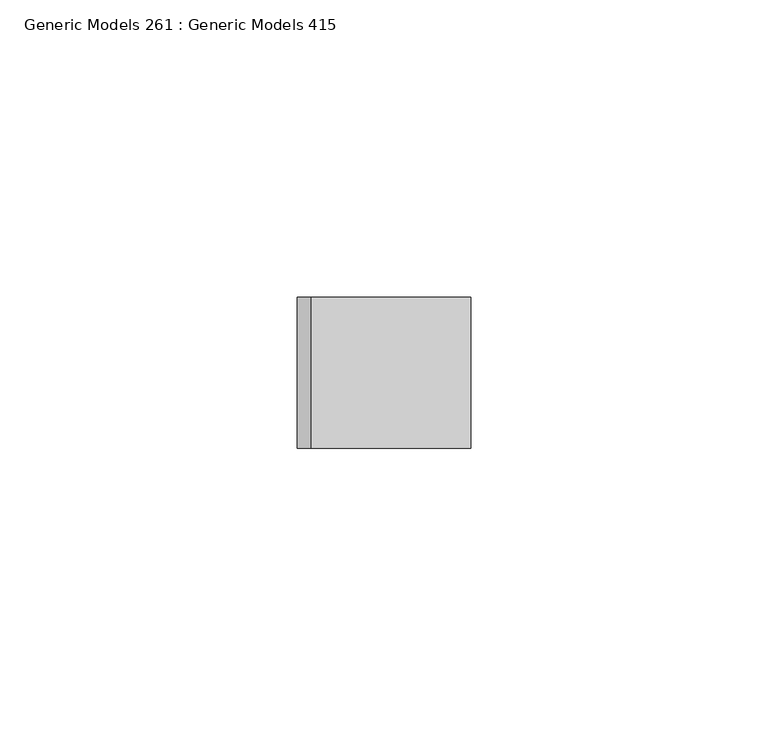
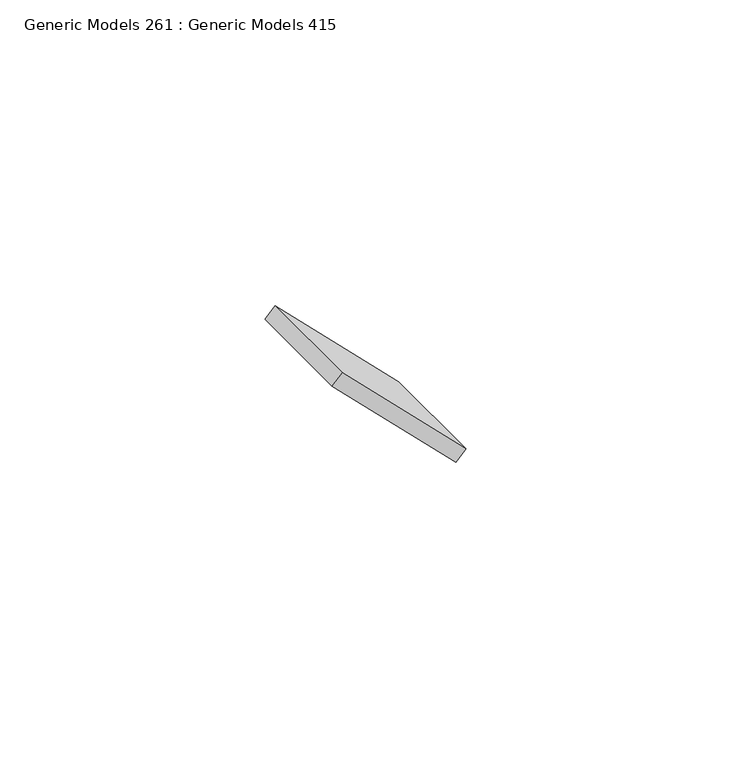
"""IFC4 building model written with IfcOpenShell, lengths in millimetres: proxy geometry, Generic Models 261 : Generic Models 415."""

import ifcopenshell
import ifcopenshell.guid

model = None  # the IFC model being written
_history = None  # IfcOwnerHistory: only IFC2X3 demands one
_inside = {}  # id of a spatial element -> (the spatial element, [elements in it])
_under = {}  # id of a project, library or spatial element -> (it, [spatial elements below it])
_declared = {}  # id of a project -> (the project, [libraries it declares])
_typed = {}  # id of a type object -> (the type object, [elements of that type])
_made_of = {}  # id of a material, layer set ... -> (it, [elements and type objects made of it])


def new_model(schema):
    """Start an empty IFC model of exactly this schema.

    Asked for "IFC4X3", IfcOpenShell would pick the latest addendum, in which some entities
    have other attributes; the version numbers below select the first issue.
    IFC2X3 requires an IfcOwnerHistory on every rooted entity: one is made here for all.
    """
    global model, _history
    if schema == "IFC4X3":
        model = ifcopenshell.file(schema_version=(4, 3, 0, 0))
    else:
        model = ifcopenshell.file(schema=schema)
    _inside.clear()
    _under.clear()
    _declared.clear()
    _typed.clear()
    _made_of.clear()
    _history = None
    if model.schema == "IFC2X3":
        org = make("IfcOrganization", Name="unknown")
        user = make(
            "IfcPersonAndOrganization",
            ThePerson=make("IfcPerson", FamilyName="unknown"),
            TheOrganization=org,
        )
        app = make(
            "IfcApplication",
            ApplicationDeveloper=org,
            Version="unknown",
            ApplicationFullName="unknown",
            ApplicationIdentifier="unknown",
        )
        _history = make(
            "IfcOwnerHistory",
            OwningUser=user,
            OwningApplication=app,
            ChangeAction="ADDED",
            CreationDate=0,
        )
    return model


def make(cls, **values):
    """One entity of the class cls with the attributes given. An attribute that is None is left unset."""
    return model.create_entity(
        cls, **{name: value for name, value in values.items() if value is not None}
    )


def rooted(cls, **values):
    """An entity with a GlobalId (a new one), such as an element, a storey or a relation."""
    return make(cls, GlobalId=ifcopenshell.guid.new(), OwnerHistory=_history, **values)


def si_unit(unit_type, name, prefix=None):
    """IfcSIUnit, for example si_unit("LENGTHUNIT", "METRE", prefix="MILLI")."""
    return make("IfcSIUnit", UnitType=unit_type, Prefix=prefix, Name=name)


def assignment(units):
    """IfcUnitAssignment: the units of a project."""
    return None if units is None else make("IfcUnitAssignment", Units=units)


def point(xyz):
    """IfcCartesianPoint."""
    return None if xyz is None else make("IfcCartesianPoint", Coordinates=xyz)


def direction(xyz):
    """IfcDirection."""
    return None if xyz is None else make("IfcDirection", DirectionRatios=xyz)


def frame(location, z_axis=None, x_axis=None):
    """IfcAxis2Placement3D, a coordinate frame: its origin and axes. An axis left out is left unset."""
    return make(
        "IfcAxis2Placement3D",
        Location=point(location),
        Axis=direction(z_axis),
        RefDirection=direction(x_axis),
    )


def origin():
    """The frame at (0, 0, 0) with its axes left unset."""
    return frame((0.0, 0.0, 0.0))


def place(relative_to, where):
    """IfcLocalPlacement: puts the frame where relative to a parent placement (None: the world)."""
    return make(
        "IfcLocalPlacement", PlacementRelTo=relative_to, RelativePlacement=where
    )


def context(
    kind, dimensions, precision=None, world=None, true_north=None, identifier=None
):
    """IfcGeometricRepresentationContext, for example the 3D "Model" context."""
    return make(
        "IfcGeometricRepresentationContext",
        ContextIdentifier=identifier,
        ContextType=kind,
        CoordinateSpaceDimension=dimensions,
        Precision=precision,
        WorldCoordinateSystem=world,
        TrueNorth=true_north,
    )


def project(units=None, contexts=None):
    """IfcProject with its units and contexts."""
    return rooted(
        "IfcProject",
        Name="project",
        RepresentationContexts=contexts,
        UnitsInContext=assignment(units),
    )


def spatial(cls, under=None, at=None, **own):
    """A site, building, storey or space (cls), placed at a placement, below another one or the project."""
    s = rooted(cls, ObjectPlacement=at, **own)
    if under is not None:
        _under.setdefault(under.id(), (under, []))[1].append(s)
    return s


def polyline(points):
    """IfcPolyline through the points."""
    return make("IfcPolyline", Points=[point(p) for p in points])


def outline(outer, holes=None, kind="AREA"):
    """IfcArbitraryClosedProfileDef: a profile drawn as a closed curve; with holes, ...WithVoids."""
    if holes is None:
        return make("IfcArbitraryClosedProfileDef", ProfileType=kind, OuterCurve=outer)
    return make(
        "IfcArbitraryProfileDefWithVoids",
        ProfileType=kind,
        OuterCurve=outer,
        InnerCurves=holes,
    )


def extrude(swept, where, along, depth):
    """IfcExtrudedAreaSolid: the profile swept, set in the frame where, extruded along a direction by depth."""
    return make(
        "IfcExtrudedAreaSolid",
        SweptArea=swept,
        Position=where,
        ExtrudedDirection=direction(along),
        Depth=depth,
    )


def shape(context_of_items, identifier, shape_type, items):
    """IfcShapeRepresentation: the items that make up one representation, for example the "Body"."""
    return make(
        "IfcShapeRepresentation",
        ContextOfItems=context_of_items,
        RepresentationIdentifier=identifier,
        RepresentationType=shape_type,
        Items=items,
    )


def source(mapping_origin, context_of_items, identifier, shape_type, items):
    """IfcRepresentationMap: a shape defined once, which mapped items show again and again."""
    return make(
        "IfcRepresentationMap",
        MappingOrigin=mapping_origin,
        MappedRepresentation=shape(context_of_items, identifier, shape_type, items),
    )


def transform(
    local_origin,
    x_axis=None,
    y_axis=None,
    z_axis=None,
    scale=None,
    scale2=None,
    scale3=None,
    uniform=True,
):
    """IfcCartesianTransformationOperator3D, or its non-uniform kind. x_axis, y_axis, z_axis: its Axis1, 2, 3."""
    if uniform:
        return make(
            "IfcCartesianTransformationOperator3D",
            Axis1=direction(x_axis),
            Axis2=direction(y_axis),
            LocalOrigin=point(local_origin),
            Scale=scale,
            Axis3=direction(z_axis),
        )
    return make(
        "IfcCartesianTransformationOperator3DnonUniform",
        Axis1=direction(x_axis),
        Axis2=direction(y_axis),
        LocalOrigin=point(local_origin),
        Scale=scale,
        Axis3=direction(z_axis),
        Scale2=scale2,
        Scale3=scale3,
    )


def mapped(mapping_source, mapping_target):
    """IfcMappedItem: shows the shape of a source again, moved by a transform."""
    return make(
        "IfcMappedItem", MappingSource=mapping_source, MappingTarget=mapping_target
    )


def made_of(thing, what):
    """Note that an element or type object is made of a material, layer set ...; save() writes the relation."""
    if what is not None:
        _made_of.setdefault(what.id(), (what, []))[1].append(thing)
    return thing


def element(
    cls,
    number,
    at=None,
    inside=None,
    cuts=None,
    type_object=None,
    material=None,
    context=None,
    identifier="Body",
    shape_type=None,
    held_by="IfcProductDefinitionShape",
    body=None,
    shapes=None,
    **own,
):
    """One element of the class cls, such as IfcWall. Its Tag is "e" and its number.

    at: its placement. inside: the storey or other place that contains it. cuts: it is an
    opening in that element (IfcRelVoidsElement). A single representation is given by context,
    identifier, shape_type and body (its items); several are given by shapes. held_by: the class
    of the entity that holds the representations. save() writes the other relations.
    """
    e = rooted(cls, Tag="e%d" % number, ObjectPlacement=at, **own)
    if body is not None:
        shapes = [shape(context, identifier, shape_type, body)]
    if shapes is not None:
        e.Representation = make(held_by, Representations=shapes)
    if inside is not None:
        _inside.setdefault(inside.id(), (inside, []))[1].append(e)
    if cuts is not None:
        rooted(
            "IfcRelVoidsElement", RelatingBuildingElement=cuts, RelatedOpeningElement=e
        )
    if type_object is not None:
        _typed.setdefault(type_object.id(), (type_object, []))[1].append(e)
    return made_of(e, material)


def aggregate(whole, parts):
    """IfcRelAggregates: a whole, such as a stair, and the parts it consists of."""
    return rooted("IfcRelAggregates", RelatingObject=whole, RelatedObjects=parts)


def save(model, path):
    """Write the relations noted so far, then the file.

    IfcRelAggregates (storeys below a building ...), IfcRelContainedInSpatialStructure (elements
    in a storey), IfcRelDefinesByType, IfcRelAssociatesMaterial and IfcRelDeclares: one each for
    every whole, place, type object, material and project.
    """
    for whole, parts in _under.values():
        aggregate(whole, parts)
    for where, things in _inside.values():
        rooted(
            "IfcRelContainedInSpatialStructure",
            RelatedElements=things,
            RelatingStructure=where,
        )
    for kind, things in _typed.values():
        rooted("IfcRelDefinesByType", RelatedObjects=things, RelatingType=kind)
    for what, things in _made_of.values():
        rooted("IfcRelAssociatesMaterial", RelatedObjects=things, RelatingMaterial=what)
    for by, libraries in _declared.values():
        rooted("IfcRelDeclares", RelatingContext=by, RelatedDefinitions=libraries)
    model.write(path)


def generic_models_261_generic_models_415_7123ed22(model_context):
    return source(origin(), model_context, "Body", "SweptSolid", [
        extrude(outline(polyline([(0.0, -38.1), (0.0, 0.0), (25.4, 0.0), (25.4, -38.1), (0.0, -38.1)])), frame((-6869.8996186, -4475.9863946, 128353.0002957), z_axis=(0.7071067811864907, 0.0, 0.7071067811866044), x_axis=(0.0, -1.0, 0.0)), (0.0, 0.0, 1.0), 3.175),
    ])


if __name__ == "__main__":
    model = new_model("IFC4")
    model_context = context("Model", 3, world=origin())
    ifc_project = project(units=[si_unit("LENGTHUNIT", "METRE", prefix="MILLI")], contexts=[model_context])
    site = spatial("IfcSite", under=ifc_project)
    building = spatial("IfcBuilding", under=site)
    placement = place(None, origin())
    generic_models_261_generic_models_415_shape = generic_models_261_generic_models_415_7123ed22(model_context)
    element("IfcBuildingElementProxy", 1, Name="Generic Models 261 : Generic Models 415", ObjectType="Generic Models 261 : Generic Models 415", at=placement, inside=building, context=model_context, shape_type="MappedRepresentation", body=[
        mapped(generic_models_261_generic_models_415_shape, transform((0.0, 0.0, 0.0), x_axis=(1.0, 0.0, 0.0), y_axis=(0.0, 1.0, 0.0), z_axis=(0.0, 0.0, 1.0))),
    ])
    save(model, "model.ifc")

# Revit data of these elements
# Element 1 (IfcBuildingElementProxy, "Generic Models 261 : Generic Models 415")
#   Materials on its faces: "_WELDED STEEL TABS FOR LOUVER ATTACHMENT"
# Materials
#   "_WELDED STEEL TABS FOR LOUVER ATTACHMENT": class "Metal", colour RGB 199 199 199, transparency 0, Description = "Structural steel 50ksi", Cost = 0
